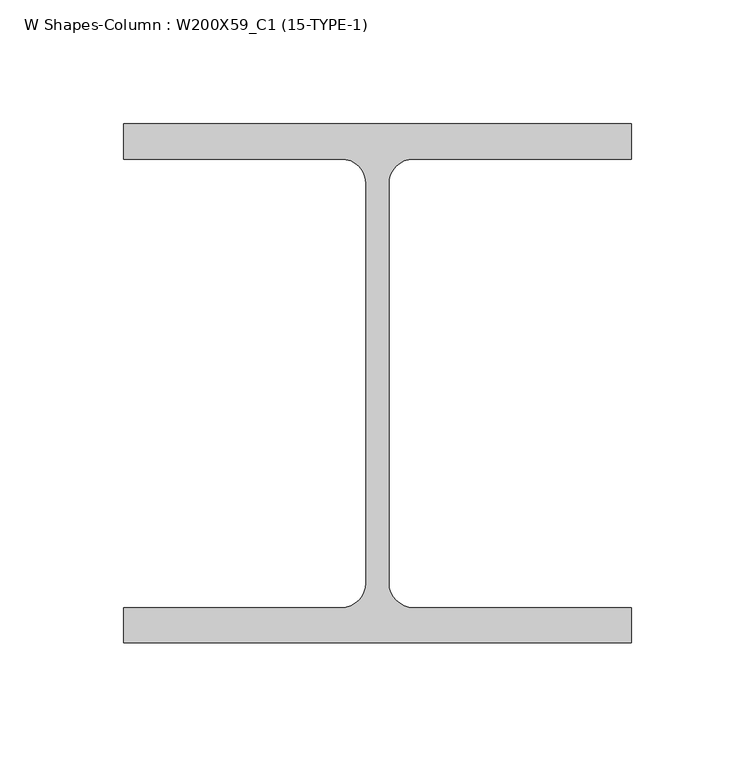
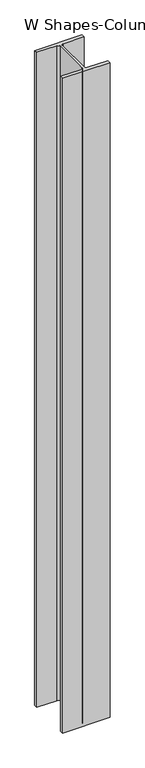
"""IFC4 building model written with IfcOpenShell, lengths in millimetres: column geometry, W Shapes-Column : W200X59_C1 (15-TYPE-1)."""

from ifc_helpers import new_model, si_unit, point, frame, frame_2d, origin, place, context, project, spatial, polyline, circle_curve, trimmed, segment, composite_curve, outline, extrude, source, transform, mapped, element, save


def w_shapes_column_w200x59_c1_15_type_1_29706d8c(model_context):
    return source(origin(), model_context, "Body", "SweptSolid", [
        extrude(outline(composite_curve([segment(polyline([(102.489, 104.775), (102.489, 90.551), (14.5796, 90.551)]), True, "CONTINUOUS"), segment(trimmed(circle_curve(frame_2d((14.5796, 80.5434)), 10.0076), [point((14.5796, 90.551))], [point((4.572, 80.5434))], True, "CARTESIAN"), True, "CONTINUOUS"), segment(polyline([(4.572, 80.5434), (4.572, -80.5434)]), True, "CONTINUOUS"), segment(trimmed(circle_curve(frame_2d((14.5796, -80.5434)), 10.0076), [point((4.572, -80.5434))], [point((14.5796, -90.551))], True, "CARTESIAN"), True, "CONTINUOUS"), segment(polyline([(14.5796, -90.551), (102.489, -90.551), (102.489, -104.775), (-102.489, -104.775), (-102.489, -90.551), (-14.5796, -90.551)]), True, "CONTINUOUS"), segment(trimmed(circle_curve(frame_2d((-14.5796, -80.5434)), 10.0076), [point((-14.5796, -90.551))], [point((-4.572, -80.5434))], True, "CARTESIAN"), True, "CONTINUOUS"), segment(polyline([(-4.572, -80.5434), (-4.572, 80.5434)]), True, "CONTINUOUS"), segment(trimmed(circle_curve(frame_2d((-14.5796, 80.5434)), 10.0076), [point((-4.572, 80.5434))], [point((-14.5796, 90.551))], True, "CARTESIAN"), True, "CONTINUOUS"), segment(polyline([(-14.5796, 90.551), (-102.489, 90.551), (-102.489, 104.775), (102.489, 104.775)]), True, "CONTINUOUS")], self_intersect=False)), frame((0.0, 0.0, 9760.0), z_axis=(0.0, 0.0, 1.0), x_axis=(1.0, 0.0, 0.0)), (0.0, 0.0, 1.0), 3000.0),
    ])


if __name__ == "__main__":
    model = new_model("IFC4")
    model_context = context("Model", 3, world=origin())
    ifc_project = project(units=[si_unit("LENGTHUNIT", "METRE", prefix="MILLI")], contexts=[model_context])
    site = spatial("IfcSite", under=ifc_project)
    building = spatial("IfcBuilding", under=site)
    placement = place(None, origin())
    w_shapes_column_w200x59_c1_15_type_1_shape = w_shapes_column_w200x59_c1_15_type_1_29706d8c(model_context)
    element("IfcColumn", 1, ObjectType="W Shapes-Column : W200X59_C1 (15-TYPE-1)", at=placement, inside=building, context=model_context, shape_type="MappedRepresentation", body=[
        mapped(w_shapes_column_w200x59_c1_15_type_1_shape, transform((0.0, 0.0, 0.0), x_axis=(1.0, 0.0, 0.0), y_axis=(0.0, 1.0, 0.0), z_axis=(0.0, 0.0, 1.0))),
    ])
    save(model, "model.ifc")

# Revit data of these elements
# Type "W Shapes-Column : W200X59_C1 (15-TYPE-1)"
#   Section Name Key = "W8x40"
#   Assembly Code = "B10"
#   Width = 20.4978 cm
#   Web Thickness = 0.9144 cm
#   Web Fillet = 1.0008 cm
#   Warping Constant = 194957.0 cm⁶
#   Torsional Moment of Inertia = 46.6179 cm⁴
#   Section Area = 75.4837 cm²
#   Plastic Modulus weak axis = 303.161 cm³
#   Plastic Modulus strong axis = 652.205 cm³
#   Perimeter = 1.20396 m²/m
#   Nominal Weight = 59.5266 kgf/m
#   Moment of Inertia weak axis = 2043.70 cm⁴
#   Moment of Inertia strong axis = 6076.98 cm⁴
#   Height = 20.955 cm
#   Flange Thickness = 1.4224 cm
#   Elastic Modulus weak axis = 199.922 cm³
#   Elastic Modulus strong axis = 581.741 cm³
#   Clear Web Height = 19.05 cm
#   Centroid Vertical = 10.4775 cm
#   Centroid Horizontal = 10.2489 cm
#   Bolt Spacing = 13.97 cm
#   Structural Material [instance default] = Steel ASTM A992
#   Principal Axes Angle = 0
# Element 1 (IfcColumn, "W Shapes-Column : W200X59_C1 (15-TYPE-1)")
#   Structural Material = none
# Materials
#   "Steel ASTM A992": class "Metal", colour RGB 199 199 199, transparency 0, Description = "Structural steel 50ksi", Cost = 0
